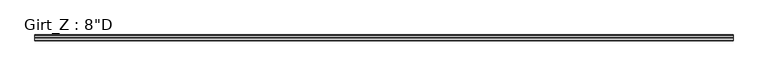
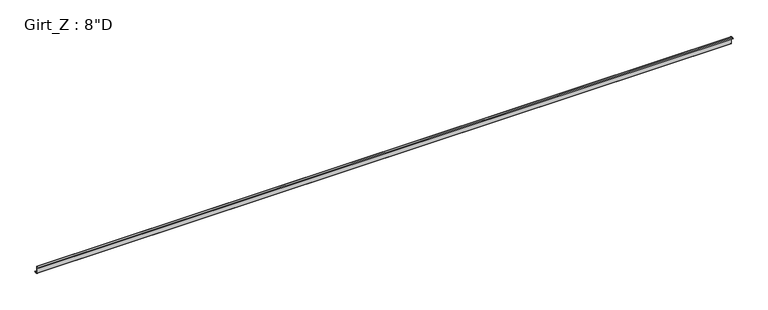
"""IFC4 building model written with IfcOpenShell, lengths in millimetres: beam geometry."""

from ifc_helpers import new_model, si_unit, point, frame, frame_2d, origin, place, context, project, spatial, polyline, circle_curve, trimmed, segment, composite_curve, outline, extrude, source, transform, mapped, element, save


def beam_7c8f2e1c(model_context):
    return source(origin(), model_context, "Body", "SweptSolid", [
        extrude(outline(composite_curve([segment(polyline([(-63.5, 101.6), (-3.3734375, 101.6)]), True, "CONTINUOUS"), segment(trimmed(circle_curve(frame_2d((-3.3734375, 96.8375)), 4.7625), [point((-3.3734375, 101.6))], [point((1.3890625, 96.8375))], False, "CARTESIAN"), True, "CONTINUOUS"), segment(polyline([(1.3890625, 96.8375), (1.3890625, -96.8389339)]), True, "CONTINUOUS"), segment(trimmed(circle_curve(frame_2d((3.3748024, -96.8389339)), 1.9857399), [point((1.3890625, -96.8389339))], [point((3.2694106, -98.821875))], True, "CARTESIAN"), True, "CONTINUOUS"), segment(polyline([(3.2694106, -98.821875), (62.204539, -98.821875), (73.6169367, -85.221109), (75.745104, -87.0068534), (63.5, -101.6), (3.3734375, -101.6)]), True, "CONTINUOUS"), segment(trimmed(circle_curve(frame_2d((3.3734375, -96.8375)), 4.7625), [point((3.3734375, -101.6))], [point((-1.3890625, -96.8375))], False, "CARTESIAN"), True, "CONTINUOUS"), segment(polyline([(-1.3890625, -96.8375), (-1.3890625, 96.8381931)]), True, "CONTINUOUS"), segment(trimmed(circle_curve(frame_2d((-3.3741066, 96.8381931)), 1.9850441), [point((-1.3890625, 96.8381931))], [point((-3.3005807, 98.821875))], True, "CARTESIAN"), True, "CONTINUOUS"), segment(polyline([(-3.3005807, 98.821875), (-62.204539, 98.821875), (-73.6169367, 85.221109), (-75.745104, 87.0068534), (-63.5, 101.6)]), True, "CONTINUOUS")], self_intersect=False)), frame((-9209.8316406, 0.0, 0.0), z_axis=(1.0, 0.0, 0.0), x_axis=(0.0, 1.0, 0.0)), (0.0, 0.0, 1.0), 18529.7960937),
    ])


if __name__ == "__main__":
    model = new_model("IFC4")
    model_context = context("Model", 3, world=origin())
    ifc_project = project(units=[si_unit("LENGTHUNIT", "METRE", prefix="MILLI")], contexts=[model_context])
    site = spatial("IfcSite", under=ifc_project)
    building = spatial("IfcBuilding", under=site)
    placement = place(None, origin())
    beam_shape = beam_7c8f2e1c(model_context)
    element("IfcBeam", 1, ObjectType="Girt_Z : 8\"D", at=placement, inside=building, context=model_context, shape_type="MappedRepresentation", body=[
        mapped(beam_shape, transform((0.0, 0.0, 0.0), x_axis=(1.0, 0.0, 0.0), y_axis=(0.0, 1.0, 0.0), z_axis=(0.0, 0.0, 1.0))),
    ])
    save(model, "model.ifc")

# Revit data of these elements
# Type "Girt_Z : 8\"D"
#   Web_Thickness = 0' - 0 7/64"
#   Length [instance default] = 10' - 0"
#   Leg_1 = 0' - 2 1/2"
#   Height = 0' - 8"
#   Structural Material [instance default] = none
# Element 1 (IfcBeam, "Girt_Z : 8\"D")
#   Structural Material = Steel
#   Materials on its faces: "Steel"
# Materials
#   "Steel": class "Metal", colour RGB 118 118 114, transparency 0, Description = "Steel, mill finish", Cost = 0
